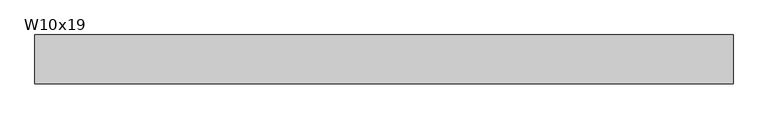
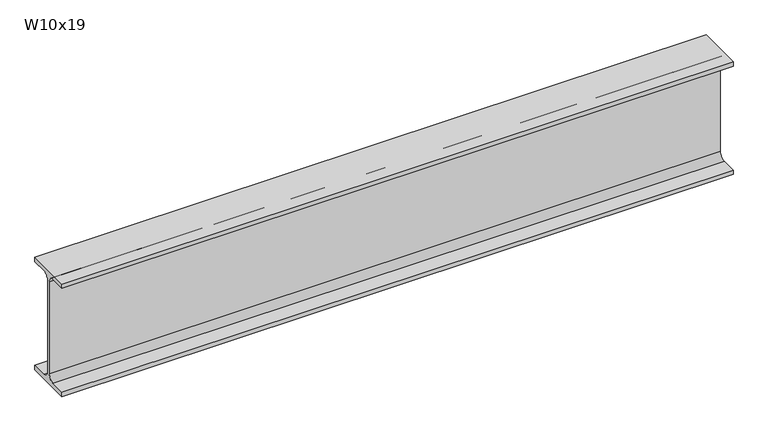
"""IFC4 building model written with IfcOpenShell, lengths in millimetres: beam geometry, RME W-Wide Flange : W10x19."""

from ifc_helpers import new_model, si_unit, point, frame, frame_2d, origin, place, context, project, spatial, polyline, circle_curve, trimmed, segment, composite_curve, outline, extrude, source, transform, mapped, element, save


def w10x19_a762532e(model_context):
    return source(origin(), model_context, "Body", "SweptSolid", [
        extrude(outline(composite_curve([segment(polyline([(51.054, -119.507), (51.054, -129.54), (-51.054, -129.54), (-51.054, -119.507), (-16.9545, -119.507)]), True, "CONTINUOUS"), segment(trimmed(circle_curve(frame_2d((-16.9545, -105.7275)), 13.7795), [point((-16.9545, -119.507))], [point((-3.175, -105.7275))], True, "CARTESIAN"), True, "CONTINUOUS"), segment(polyline([(-3.175, -105.7275), (-3.175, 105.7275)]), True, "CONTINUOUS"), segment(trimmed(circle_curve(frame_2d((-16.9545, 105.7275)), 13.7795), [point((-3.175, 105.7275))], [point((-16.9545, 119.507))], True, "CARTESIAN"), True, "CONTINUOUS"), segment(polyline([(-16.9545, 119.507), (-51.054, 119.507), (-51.054, 129.54), (51.054, 129.54), (51.054, 119.507), (16.9545, 119.507)]), True, "CONTINUOUS"), segment(trimmed(circle_curve(frame_2d((16.9545, 105.7275)), 13.7795), [point((16.9545, 119.507))], [point((3.175, 105.7275))], True, "CARTESIAN"), True, "CONTINUOUS"), segment(polyline([(3.175, 105.7275), (3.175, -105.7275)]), True, "CONTINUOUS"), segment(trimmed(circle_curve(frame_2d((16.9545, -105.7275)), 13.7795), [point((3.175, -105.7275))], [point((16.9545, -119.507))], True, "CARTESIAN"), True, "CONTINUOUS"), segment(polyline([(16.9545, -119.507), (51.054, -119.507)]), True, "CONTINUOUS")], self_intersect=False)), frame((-698.416953, 0.0, 0.0), z_axis=(1.0, 0.0, 0.0), x_axis=(0.0, 1.0, 0.0)), (0.0, 0.0, 1.0), 1460.5771735),
    ])


if __name__ == "__main__":
    model = new_model("IFC4")
    model_context = context("Model", 3, world=origin())
    ifc_project = project(units=[si_unit("LENGTHUNIT", "METRE", prefix="MILLI")], contexts=[model_context])
    site = spatial("IfcSite", under=ifc_project)
    building = spatial("IfcBuilding", under=site)
    placement = place(None, origin())
    w10x19_shape = w10x19_a762532e(model_context)
    element("IfcBeam", 1, ObjectType="RME W-Wide Flange : W10x19", at=placement, inside=building, context=model_context, shape_type="MappedRepresentation", body=[
        mapped(w10x19_shape, transform((0.0, 0.0, 0.0), x_axis=(1.0, 0.0, 0.0), y_axis=(0.0, 1.0, 0.0), z_axis=(0.0, 0.0, 1.0))),
    ])
    save(model, "model.ifc")

# Revit data of these elements
# Type "RME W-Wide Flange : W10x19"
#   WELD P [instance default] = ""
#   WELD LE [instance default] = ""
#   WELD D [instance default] = ""
#   TOP SECTION SIZE [instance default] = ""
#   TOP SECTION LENGTH [instance default] = ""
#   REMARKS [instance default] = ""
#   REINF TYPE [instance default] = ""
#   Nominal Size = "W24"
#   End Bearing Capacity [instance default] = ""
#   BOT SECTION SIZE [instance default] = ""
#   BOT SECTION LENGTH [instance default] = ""
#   Assembly Code = "B10"
#   W = 19
#   Start Extension Calculation [instance default] = 10' - 0"
#   Start Extension [instance default] = -0' - 0 1/2"
#   End Extension Calculation [instance default] = 10' - 0"
#   End Extension [instance default] = -0' - 0 1/2"
#   Length [instance default] = 5' - 0"
#   bf = 0' - 4.02"
#   d = 0' - 10.2"
#   k = 0' - 0 15/16"
#   k2 = 0' - 0.5425"
#   tf = 0' - 0.395"
#   tw = 0' - 0 1/4"
#   A = 0.0390278 SF
#   Structural Material [instance default] = Metal - Steel - ASTM A992
# Element 1 (IfcBeam, "RME W-Wide Flange : W10x19")
#   Length = 5' - 0.01262"
#   Materials on its faces: "Metal - Steel - ASTM A992"
# Materials
#   "Metal - Steel - ASTM A992": class "Metal", colour RGB 255 128 0, transparency 0
